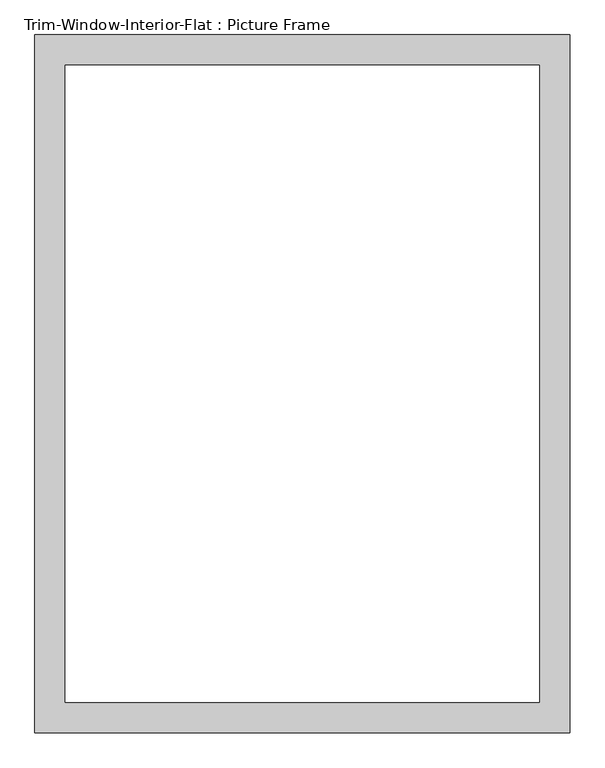
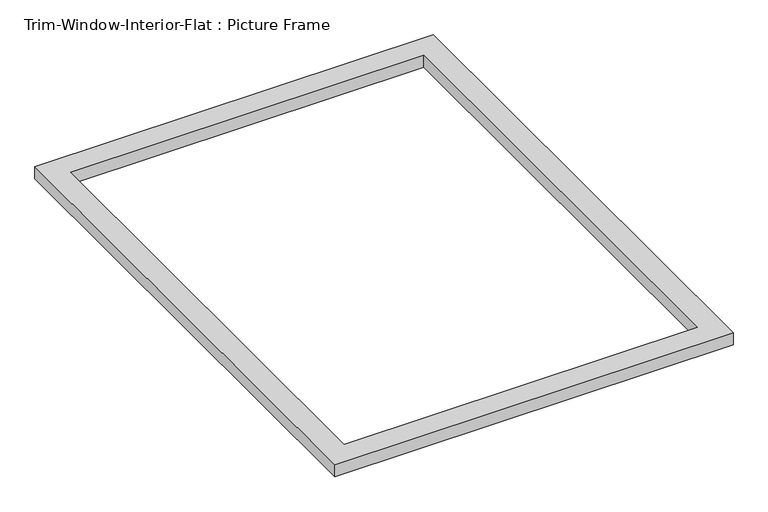
"""IFC4 building model written with IfcOpenShell, lengths in millimetres: proxy geometry, Trim-Window-Interior-Flat : Picture Frame."""

import ifcopenshell
import ifcopenshell.guid

model = None  # the IFC model being written
_history = None  # IfcOwnerHistory: only IFC2X3 demands one
_inside = {}  # id of a spatial element -> (the spatial element, [elements in it])
_under = {}  # id of a project, library or spatial element -> (it, [spatial elements below it])
_declared = {}  # id of a project -> (the project, [libraries it declares])
_typed = {}  # id of a type object -> (the type object, [elements of that type])
_made_of = {}  # id of a material, layer set ... -> (it, [elements and type objects made of it])


def new_model(schema):
    """Start an empty IFC model of exactly this schema.

    Asked for "IFC4X3", IfcOpenShell would pick the latest addendum, in which some entities
    have other attributes; the version numbers below select the first issue.
    IFC2X3 requires an IfcOwnerHistory on every rooted entity: one is made here for all.
    """
    global model, _history
    if schema == "IFC4X3":
        model = ifcopenshell.file(schema_version=(4, 3, 0, 0))
    else:
        model = ifcopenshell.file(schema=schema)
    _inside.clear()
    _under.clear()
    _declared.clear()
    _typed.clear()
    _made_of.clear()
    _history = None
    if model.schema == "IFC2X3":
        org = make("IfcOrganization", Name="unknown")
        user = make(
            "IfcPersonAndOrganization",
            ThePerson=make("IfcPerson", FamilyName="unknown"),
            TheOrganization=org,
        )
        app = make(
            "IfcApplication",
            ApplicationDeveloper=org,
            Version="unknown",
            ApplicationFullName="unknown",
            ApplicationIdentifier="unknown",
        )
        _history = make(
            "IfcOwnerHistory",
            OwningUser=user,
            OwningApplication=app,
            ChangeAction="ADDED",
            CreationDate=0,
        )
    return model


def make(cls, **values):
    """One entity of the class cls with the attributes given. An attribute that is None is left unset."""
    return model.create_entity(
        cls, **{name: value for name, value in values.items() if value is not None}
    )


def rooted(cls, **values):
    """An entity with a GlobalId (a new one), such as an element, a storey or a relation."""
    return make(cls, GlobalId=ifcopenshell.guid.new(), OwnerHistory=_history, **values)


def si_unit(unit_type, name, prefix=None):
    """IfcSIUnit, for example si_unit("LENGTHUNIT", "METRE", prefix="MILLI")."""
    return make("IfcSIUnit", UnitType=unit_type, Prefix=prefix, Name=name)


def assignment(units):
    """IfcUnitAssignment: the units of a project."""
    return None if units is None else make("IfcUnitAssignment", Units=units)


def point(xyz):
    """IfcCartesianPoint."""
    return None if xyz is None else make("IfcCartesianPoint", Coordinates=xyz)


def direction(xyz):
    """IfcDirection."""
    return None if xyz is None else make("IfcDirection", DirectionRatios=xyz)


def frame(location, z_axis=None, x_axis=None):
    """IfcAxis2Placement3D, a coordinate frame: its origin and axes. An axis left out is left unset."""
    return make(
        "IfcAxis2Placement3D",
        Location=point(location),
        Axis=direction(z_axis),
        RefDirection=direction(x_axis),
    )


def origin():
    """The frame at (0, 0, 0) with its axes left unset."""
    return frame((0.0, 0.0, 0.0))


def origin_with_axes():
    """The frame at (0, 0, 0) with the z axis (0, 0, 1) and the x axis (1, 0, 0) written out."""
    return frame((0.0, 0.0, 0.0), z_axis=(0.0, 0.0, 1.0), x_axis=(1.0, 0.0, 0.0))


def place(relative_to, where):
    """IfcLocalPlacement: puts the frame where relative to a parent placement (None: the world)."""
    return make(
        "IfcLocalPlacement", PlacementRelTo=relative_to, RelativePlacement=where
    )


def context(
    kind, dimensions, precision=None, world=None, true_north=None, identifier=None
):
    """IfcGeometricRepresentationContext, for example the 3D "Model" context."""
    return make(
        "IfcGeometricRepresentationContext",
        ContextIdentifier=identifier,
        ContextType=kind,
        CoordinateSpaceDimension=dimensions,
        Precision=precision,
        WorldCoordinateSystem=world,
        TrueNorth=true_north,
    )


def project(units=None, contexts=None):
    """IfcProject with its units and contexts."""
    return rooted(
        "IfcProject",
        Name="project",
        RepresentationContexts=contexts,
        UnitsInContext=assignment(units),
    )


def spatial(cls, under=None, at=None, **own):
    """A site, building, storey or space (cls), placed at a placement, below another one or the project."""
    s = rooted(cls, ObjectPlacement=at, **own)
    if under is not None:
        _under.setdefault(under.id(), (under, []))[1].append(s)
    return s


def polyline(points):
    """IfcPolyline through the points."""
    return make("IfcPolyline", Points=[point(p) for p in points])


def outline(outer, holes=None, kind="AREA"):
    """IfcArbitraryClosedProfileDef: a profile drawn as a closed curve; with holes, ...WithVoids."""
    if holes is None:
        return make("IfcArbitraryClosedProfileDef", ProfileType=kind, OuterCurve=outer)
    return make(
        "IfcArbitraryProfileDefWithVoids",
        ProfileType=kind,
        OuterCurve=outer,
        InnerCurves=holes,
    )


def extrude(swept, where, along, depth):
    """IfcExtrudedAreaSolid: the profile swept, set in the frame where, extruded along a direction by depth."""
    return make(
        "IfcExtrudedAreaSolid",
        SweptArea=swept,
        Position=where,
        ExtrudedDirection=direction(along),
        Depth=depth,
    )


def shape(context_of_items, identifier, shape_type, items):
    """IfcShapeRepresentation: the items that make up one representation, for example the "Body"."""
    return make(
        "IfcShapeRepresentation",
        ContextOfItems=context_of_items,
        RepresentationIdentifier=identifier,
        RepresentationType=shape_type,
        Items=items,
    )


def source(mapping_origin, context_of_items, identifier, shape_type, items):
    """IfcRepresentationMap: a shape defined once, which mapped items show again and again."""
    return make(
        "IfcRepresentationMap",
        MappingOrigin=mapping_origin,
        MappedRepresentation=shape(context_of_items, identifier, shape_type, items),
    )


def transform(
    local_origin,
    x_axis=None,
    y_axis=None,
    z_axis=None,
    scale=None,
    scale2=None,
    scale3=None,
    uniform=True,
):
    """IfcCartesianTransformationOperator3D, or its non-uniform kind. x_axis, y_axis, z_axis: its Axis1, 2, 3."""
    if uniform:
        return make(
            "IfcCartesianTransformationOperator3D",
            Axis1=direction(x_axis),
            Axis2=direction(y_axis),
            LocalOrigin=point(local_origin),
            Scale=scale,
            Axis3=direction(z_axis),
        )
    return make(
        "IfcCartesianTransformationOperator3DnonUniform",
        Axis1=direction(x_axis),
        Axis2=direction(y_axis),
        LocalOrigin=point(local_origin),
        Scale=scale,
        Axis3=direction(z_axis),
        Scale2=scale2,
        Scale3=scale3,
    )


def mapped(mapping_source, mapping_target):
    """IfcMappedItem: shows the shape of a source again, moved by a transform."""
    return make(
        "IfcMappedItem", MappingSource=mapping_source, MappingTarget=mapping_target
    )


def made_of(thing, what):
    """Note that an element or type object is made of a material, layer set ...; save() writes the relation."""
    if what is not None:
        _made_of.setdefault(what.id(), (what, []))[1].append(thing)
    return thing


def element(
    cls,
    number,
    at=None,
    inside=None,
    cuts=None,
    type_object=None,
    material=None,
    context=None,
    identifier="Body",
    shape_type=None,
    held_by="IfcProductDefinitionShape",
    body=None,
    shapes=None,
    **own,
):
    """One element of the class cls, such as IfcWall. Its Tag is "e" and its number.

    at: its placement. inside: the storey or other place that contains it. cuts: it is an
    opening in that element (IfcRelVoidsElement). A single representation is given by context,
    identifier, shape_type and body (its items); several are given by shapes. held_by: the class
    of the entity that holds the representations. save() writes the other relations.
    """
    e = rooted(cls, Tag="e%d" % number, ObjectPlacement=at, **own)
    if body is not None:
        shapes = [shape(context, identifier, shape_type, body)]
    if shapes is not None:
        e.Representation = make(held_by, Representations=shapes)
    if inside is not None:
        _inside.setdefault(inside.id(), (inside, []))[1].append(e)
    if cuts is not None:
        rooted(
            "IfcRelVoidsElement", RelatingBuildingElement=cuts, RelatedOpeningElement=e
        )
    if type_object is not None:
        _typed.setdefault(type_object.id(), (type_object, []))[1].append(e)
    return made_of(e, material)


def aggregate(whole, parts):
    """IfcRelAggregates: a whole, such as a stair, and the parts it consists of."""
    return rooted("IfcRelAggregates", RelatingObject=whole, RelatedObjects=parts)


def save(model, path):
    """Write the relations noted so far, then the file.

    IfcRelAggregates (storeys below a building ...), IfcRelContainedInSpatialStructure (elements
    in a storey), IfcRelDefinesByType, IfcRelAssociatesMaterial and IfcRelDeclares: one each for
    every whole, place, type object, material and project.
    """
    for whole, parts in _under.values():
        aggregate(whole, parts)
    for where, things in _inside.values():
        rooted(
            "IfcRelContainedInSpatialStructure",
            RelatedElements=things,
            RelatingStructure=where,
        )
    for kind, things in _typed.values():
        rooted("IfcRelDefinesByType", RelatedObjects=things, RelatingType=kind)
    for what, things in _made_of.values():
        rooted("IfcRelAssociatesMaterial", RelatedObjects=things, RelatingMaterial=what)
    for by, libraries in _declared.values():
        rooted("IfcRelDeclares", RelatingContext=by, RelatedDefinitions=libraries)
    model.write(path)


def trim_window_interior_flat_picture_frame_c1dcbb6d(model_context):
    return source(origin(), model_context, "Body", "SweptSolid", [
        extrude(outline(polyline([(501.65, -44.45), (-501.65, -44.45), (-501.65, 1263.65), (501.65, 1263.65), (501.65, -44.45)]), holes=[polyline([(444.5, 12.7), (444.5, 1206.5), (-444.5, 1206.5), (-444.5, 12.7), (444.5, 12.7)])]), origin_with_axes(), (0.0, 0.0, 1.0), 31.75),
    ])


if __name__ == "__main__":
    model = new_model("IFC4")
    model_context = context("Model", 3, world=origin())
    ifc_project = project(units=[si_unit("LENGTHUNIT", "METRE", prefix="MILLI")], contexts=[model_context])
    site = spatial("IfcSite", under=ifc_project)
    building = spatial("IfcBuilding", under=site)
    placement = place(None, origin())
    trim_window_interior_flat_picture_frame_shape = trim_window_interior_flat_picture_frame_c1dcbb6d(model_context)
    element("IfcBuildingElementProxy", 1, Name="Trim-Window-Interior-Flat : Picture Frame", ObjectType="Trim-Window-Interior-Flat : Picture Frame", at=placement, inside=building, context=model_context, shape_type="MappedRepresentation", body=[
        mapped(trim_window_interior_flat_picture_frame_shape, transform((0.0, 0.0, 0.0), x_axis=(1.0, 0.0, 0.0), y_axis=(0.0, 1.0, 0.0), z_axis=(0.0, 0.0, 1.0))),
    ])
    save(model, "model.ifc")

# Revit data of these elements
# Type "Trim-Window-Interior-Flat : Picture Frame"
#   Trim Thickness_Picture Frame = 0' - 1 1/4"
#   Trim Width = 0' - 2 1/4"
#   Trim Thickness_with Sill = 0' - 0 3/4"
#   Sill Thickness = 0' - 1 1/4"
#   Opening Width [instance default] = 2' - 0"
#   Opening Height [instance default] = 3' - 0"
#   Default Elevation = 4' - 0"
#   Sill = no
#   Picture Frame = yes
#   Trim Material [instance default] = none
# Element 1 (IfcBuildingElementProxy, "Trim-Window-Interior-Flat : Picture Frame")
#   Opening Width = 3' - 0"
#   Opening Height = 4' - 0"
#   Trim Material = Wood - Stained
#   Materials on its faces: "Wood - Stained"
# Materials
#   "Wood - Stained": class "Wood", colour RGB 224 178 126, transparency 0, Cost = 0
